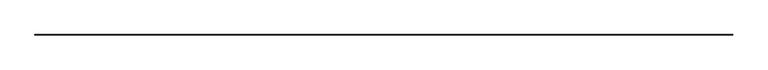
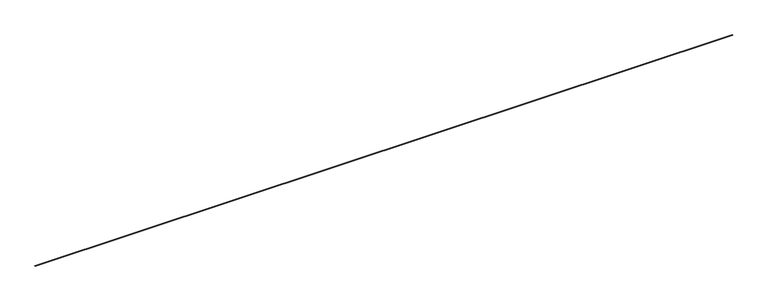
"""IFC4 building model written with IfcOpenShell, lengths in millimetres: proxy geometry, Inner panel:Inner panel:1:Inner panel:1 : Inner panel:Inner panel:300324:2:Inner panel:1:Inner panel:1 : Inner panel:Inner panel:300324:2 : Inner panel:Inner panel:1:Inner panel:1 : Inner panel:Inner panel:300324:300043:20 : Inner panel:Inner panel:1:Inner panel:1 : Inner panel:Inner panel:300324:2:Inner panel:1:Inner panel:1 : Inner panel:Inner panel:300324:2 : Inner panel:Inner panel:1:Inner panel:1 : Inner panel:Inner panel:300324:300043:308120."""

from ifc_helpers import new_model, si_unit, frame, origin, place, context, project, spatial, polyline, outline, extrude, source, transform, mapped, element, save


def generic_models_165e871d(model_context):
    return source(origin(), model_context, "Body", "SweptSolid", [
        extrude(outline(polyline([(-569678.3898252, 8703.4067109), (-569679.9759489, 8741.4736809), (-569641.9089788, 8743.0598047), (-569640.3228551, 8704.9928346), (-569678.3898252, 8703.4067109)]), holes=[polyline([(-569676.1097723, 8705.8850292), (-569642.8011734, 8707.2728875), (-569644.1890317, 8740.5814863), (-569677.4976306, 8739.1936281), (-569676.1097723, 8705.8850292)])]), frame((579104.5117239, 0.0, 0.0), z_axis=(1.0, 0.0, 0.0), x_axis=(0.0, 1.0, 0.0)), (0.0, 0.0, 1.0), 88442.8),
    ])


if __name__ == "__main__":
    model = new_model("IFC4")
    model_context = context("Model", 3, world=origin())
    ifc_project = project(units=[si_unit("LENGTHUNIT", "METRE", prefix="MILLI")], contexts=[model_context])
    site = spatial("IfcSite", under=ifc_project)
    building = spatial("IfcBuilding", under=site)
    placement = place(None, origin())
    generic_models_shape = generic_models_165e871d(model_context)
    element("IfcBuildingElementProxy", 1, Name="Inner panel:Inner panel:1:Inner panel:1 : Inner panel:Inner panel:300324:2:Inner panel:1:Inner panel:1 : Inner panel:Inner panel:300324:2 : Inner panel:Inner panel:1:Inner panel:1 : Inner panel:Inner panel:300324:300043:20 : Inner panel:Inner panel:1:Inner panel:1 : Inner panel:Inner panel:300324:2:Inner panel:1:Inner panel:1 : Inner panel:Inner panel:300324:2 : Inner panel:Inner panel:1:Inner panel:1 : Inner panel:Inner panel:300324:300043:308120", ObjectType="Inner panel:Inner panel:1:Inner panel:1 : Inner panel:Inner panel:300324:2:Inner panel:1:Inner panel:1 : Inner panel:Inner panel:300324:2 : Inner panel:Inner panel:1:Inner panel:1 : Inner panel:Inner panel:300324:300043:20 : Inner panel:Inner panel:1:Inner panel:1 : Inner panel:Inner panel:300324:2:Inner panel:1:Inner panel:1 : Inner panel:Inner panel:300324:2 : Inner panel:Inner panel:1:Inner panel:1 : Inner panel:Inner panel:300324:300043:308120", at=placement, inside=building, context=model_context, shape_type="MappedRepresentation", body=[
        mapped(generic_models_shape, transform((0.0, 0.0, 0.0), x_axis=(1.0, 0.0, 0.0), y_axis=(0.0, 1.0, 0.0), z_axis=(0.0, 0.0, 1.0))),
    ])
    save(model, "model.ifc")

# Revit data of these elements
# Type "Inner panel:Inner panel:1:Inner panel:1 : Inner panel:Inner panel:300324:2:Inner panel:1:Inner panel:1 : Inner panel:Inner panel:300324:2 : Inner panel:Inner panel:1:Inner panel:1 : Inner panel:Inner panel:300324:300043:20 : Inner panel:Inner panel:1:Inner panel:1 : Inner panel:Inner panel:300324:2:Inner panel:1:Inner panel:1 : Inner panel:Inner panel:300324:2 : Inner panel:Inner panel:1:Inner panel:1 : Inner panel:Inner panel:300324:300043:308120"
#   NameOverride = "Inner panel:Inner panel:1:Inner panel:1 : Inner panel:Inner panel:300324:2:Inner panel:1:Inner panel:1 : Inner panel:Inner panel:300324:2 : Inner panel:Inner panel:1:Inner panel:1 : Inner panel:Inner panel:300324:300043:308120"
#   ObjectTypeOverride = "Inner panel:1:Inner panel:1 : Inner panel:Inner panel:300324:2 : Inner panel:Inner panel:1:Inner panel:1 : Inner panel:Inner panel:300324:300043"
#   Reference = "Inner panel"
#   Tag = "308120"
# Element 1 (IfcBuildingElementProxy, "Inner panel:Inner panel:1:Inner panel:1 : Inner panel:Inner panel:300324:2:Inner panel:1:Inner panel:1 : Inner panel:Inner panel:300324:2 : Inner panel:Inner panel:1:Inner panel:1 : Inner panel:Inner panel:300324:300043:20 : Inner panel:Inner panel:1:Inner panel:1 : Inner panel:Inner panel:300324:2:Inner panel:1:Inner panel:1 : Inner panel:Inner panel:300324:2 : Inner panel:Inner panel:1:Inner panel:1 : Inner panel:Inner panel:300324:300043:308120")
#   Materials on its faces: "1 1/2\" X 1 1/2\" x 1/8\" ALUM. TUBE (6061-T6) - (2) #16 WOOD SCREWS WITH 2.5\" EMBED AT EACH GLULAM - (1) SCREW AT ENDS"
# Materials
#   "1 1/2\" X 1 1/2\" x 1/8\" ALUM. TUBE (6061-T6) - (2) #16 WOOD SCREWS WITH 2.5\" EMBED AT EACH GLULAM - (1) SCREW AT ENDS": class "Unassigned", colour RGB 202 201 200, transparency 0, Cost = 0
